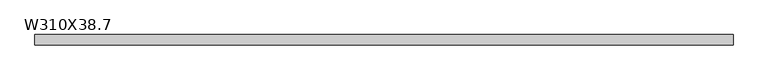
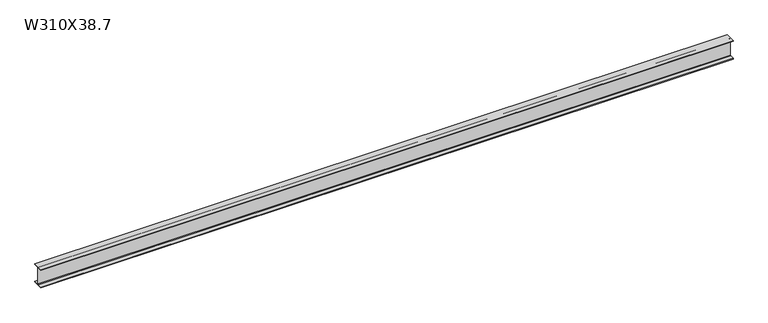
"""IFC4 building model written with IfcOpenShell, lengths in millimetres: beam geometry, M_W Shapes : W310X38.7."""

from ifc_helpers import new_model, si_unit, point, frame, frame_2d, origin, place, context, project, spatial, polyline, circle_curve, trimmed, segment, composite_curve, outline, extrude, source, transform, mapped, element, save


def w310x38_7_0f3b6658(model_context):
    return source(origin(), model_context, "Body", "SweptSolid", [
        extrude(outline(composite_curve([segment(polyline([(82.5, -145.35), (82.5, -155.0), (-82.5, -155.0), (-82.5, -145.35), (-10.57, -145.35)]), True, "CONTINUOUS"), segment(trimmed(circle_curve(frame_2d((-10.57, -137.7)), 7.65), [point((-10.57, -145.35))], [point((-2.92, -137.7))], True, "CARTESIAN"), True, "CONTINUOUS"), segment(polyline([(-2.92, -137.7), (-2.92, 137.7)]), True, "CONTINUOUS"), segment(trimmed(circle_curve(frame_2d((-10.57, 137.7)), 7.65), [point((-2.92, 137.7))], [point((-10.57, 145.35))], True, "CARTESIAN"), True, "CONTINUOUS"), segment(polyline([(-10.57, 145.35), (-82.5, 145.35), (-82.5, 155.0), (82.5, 155.0), (82.5, 145.35), (10.57, 145.35)]), True, "CONTINUOUS"), segment(trimmed(circle_curve(frame_2d((10.57, 137.7)), 7.65), [point((10.57, 145.35))], [point((2.92, 137.7))], True, "CARTESIAN"), True, "CONTINUOUS"), segment(polyline([(2.92, 137.7), (2.92, -137.7)]), True, "CONTINUOUS"), segment(trimmed(circle_curve(frame_2d((10.57, -137.7)), 7.65), [point((2.92, -137.7))], [point((10.57, -145.35))], True, "CARTESIAN"), True, "CONTINUOUS"), segment(polyline([(10.57, -145.35), (82.5, -145.35)]), True, "CONTINUOUS")], self_intersect=False)), frame((-5509.8, 0.0, 0.0), z_axis=(1.0, 0.0, 0.0), x_axis=(0.0, 1.0, 0.0)), (0.0, 0.0, 1.0), 11131.6),
    ])


if __name__ == "__main__":
    model = new_model("IFC4")
    model_context = context("Model", 3, world=origin())
    ifc_project = project(units=[si_unit("LENGTHUNIT", "METRE", prefix="MILLI")], contexts=[model_context])
    site = spatial("IfcSite", under=ifc_project)
    building = spatial("IfcBuilding", under=site)
    placement = place(None, origin())
    w310x38_7_shape = w310x38_7_0f3b6658(model_context)
    element("IfcBeam", 1, ObjectType="M_W Shapes : W310X38.7", at=placement, inside=building, context=model_context, shape_type="MappedRepresentation", body=[
        mapped(w310x38_7_shape, transform((0.0, 0.0, 0.0), x_axis=(1.0, 0.0, 0.0), y_axis=(0.0, 1.0, 0.0), z_axis=(0.0, 0.0, 1.0))),
    ])
    save(model, "model.ifc")

# Revit data of these elements
# Type "M_W Shapes : W310X38.7"
#   Section Name Key = "W12x26"
#   Width = 165 mm
#   Web Thickness = 5.84 mm
#   Web Fillet = 7.65 mm
#   Warping Constant = 163000 cm⁶
#   Torsional Moment of Inertia = 12.5 cm⁴
#   Section Area = 49.4 cm²
#   Plastic Modulus weak axis = 0.00473217 (stored number, unit not read)
#   Plastic Modulus strong axis = 0.0215419 (stored number, unit not read)
#   Perimeter = 1.25 m²/m
#   Nominal Weight = 379.516 N/m
#   Moment of Inertia weak axis = 720 cm⁴
#   Moment of Inertia strong axis = 8490 cm⁴
#   Height = 310 mm
#   Flange Thickness = 9.65 mm
#   Elastic Modulus weak axis = 0.00309003 (stored number, unit not read)
#   Elastic Modulus strong axis = 0.0193171 (stored number, unit not read)
#   Centroid Vertical = 155 mm
#   Centroid Horizontal = 82.5 mm
#   Length [instance default] = 1.5 m
#   Structural Material [instance default] = Steel, 45-345
#   Assembly Code = ""
# Element 1 (IfcBeam, "M_W Shapes : W310X38.7")
#   Materials on its faces: "Steel, 45-345"
# Materials
#   "Steel, 45-345": class "Metal", colour RGB 189 187 185, transparency 0, Description = "Steel 345 MPa", Cost = 0
